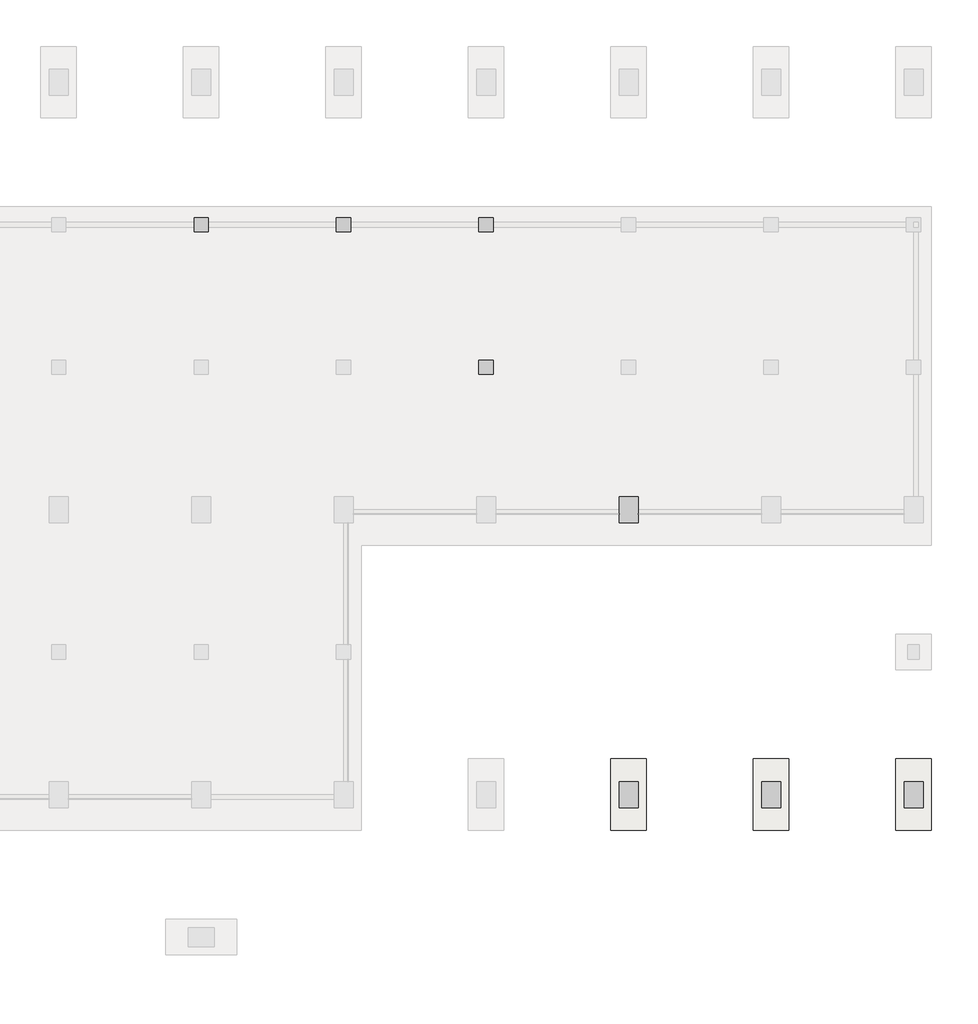
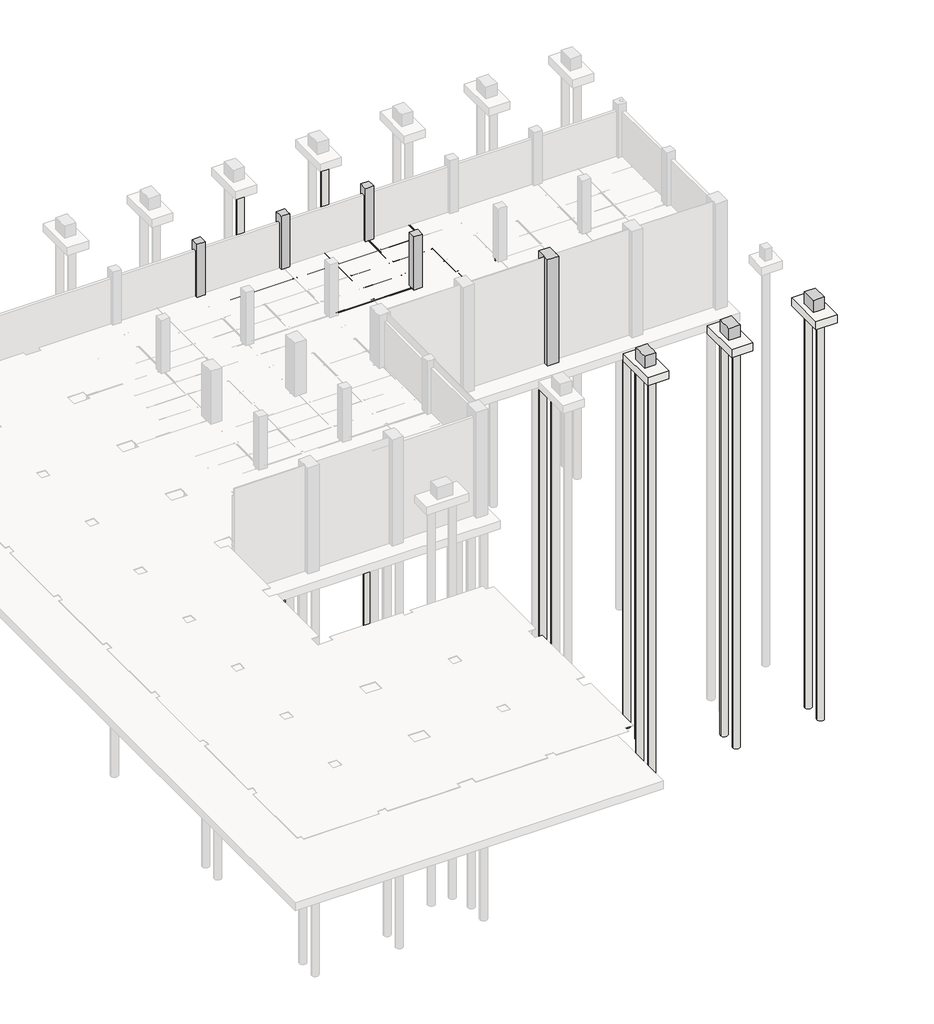
# Not in any storey, part 14 of 16: 21 beams, 17 slabs, 8 columns.
# Revit data of these elements (continued)
# Type "PILE : H_SF_AR_S19_PHC Pile_Pre-boring_D500_L30" (continued)
#   Depth = 30000 mm
#   Structural Material [instance default] = none
# Elements 1, 2, 6, 7, 8, 9, 12, 13, 14, 17, 18, 19, 20, 21 (IfcBeam, "Steel Framing_C_KS : H_SB_AR_S02_C-150x75x6.5x10_J1")
#   Structural Material = Steel, 45-345
#   Phase Created = New Construction
#   Materials on its faces: "Steel, 45-345"
# Elements 3, 10 (IfcBeam, "Steel Framing_H_KS : H_SB_AR_S02_H-400x200x8x13_BSG1")
#   Structural Material = Steel, 45-345
#   Phase Created = New Construction
#   Materials on its faces: "Steel, 45-345"
# Elements 4, 15 (IfcBeam, "Steel Framing_H_KS : H_SB_AR_S02_H-400x200x8x13_BSG2")
#   Structural Material = Steel, 45-345
#   Phase Created = New Construction
#   Materials on its faces: "Steel, 45-345"
# Elements 5, 11, 16 (IfcBeam, "Steel Framing_H_KS : H_SB_AR_S02_H-400x200x8x13_BSB1")
#   Structural Material = Steel, 45-345
#   Phase Created = New Construction
#   Materials on its faces: "Steel, 45-345"
# Elements 22, 23, 24, 25 (IfcColumn, "RC_Column_Rectangular : H_SC_AR_S15_UG PED_Bit_800x1100_PD1")
#   Comments = ""
#   hec_material3 = none
#   hec_material2 = none
#   hec_material1 = none
#   Structural Material = 00_Concrete_Reinf. Conc.
#   Phase Created = New Construction
#   Materials on its faces: "00_Concrete_Reinf. Conc."
# Elements 26, 27, 28, 29 (IfcColumn, "RC_Column_Rectangular : H_SC_AR_S15_UG PED_Bit_600x600_BC1")
#   Comments = ""
#   hec_material3 = none
#   hec_material2 = none
#   hec_material1 = none
#   Structural Material = 00_Concrete_Reinf. Conc.
#   Phase Created = New Construction
#   Materials on its faces: "00_Concrete_Reinf. Conc."
# Elements 30, 31, 32 (IfcSlab, "Foundation Rectangular (Non-Pile) : H_SF_AR_S18_Shallow Fdn_Bitumen_1500x3000xT600_F1")
#   Structural Material = 00_Concrete_Reinf. Conc.
#   Phase Created = New Construction
#   Materials on its faces: "00_Concrete_Reinf. Conc."
# Elements 33, 34, 35, 36, 37, 38, 39, 40 (IfcSlab, "PILE : H_SF_AR_S19_PHC Pile_Pre-boring_D500_L30")
#   Structural Material = Concrete, Precast
#   Phase Created = New Construction
#   Materials on its faces: "Concrete, Precast"
# Elements 41, 42, 43, 44, 45, 46 (IfcSlab, "PILE : H_SF_AR_S19_PHC Pile_Pre-boring_D500_L30")
#   Structural Material = none
#   Phase Created = New Construction
# Materials
#   "Steel, 45-345": class "Metal", colour RGB 189 187 185, transparency 0, Description = "Steel 345 MPa", Cost = 0
#   "00_Concrete_Reinf. Conc.": class "Concrete", colour RGB 176 176 176, transparency 0, Description = "Reinf. Conc.", Cost = 0, Image = Concrete.Cast-In-Place.Flat.Polished.Grey.jpg
#   "Concrete, Precast": class "Concrete", colour RGB 115 116 108, transparency 0, Description = "Precast concrete", Cost = 0
